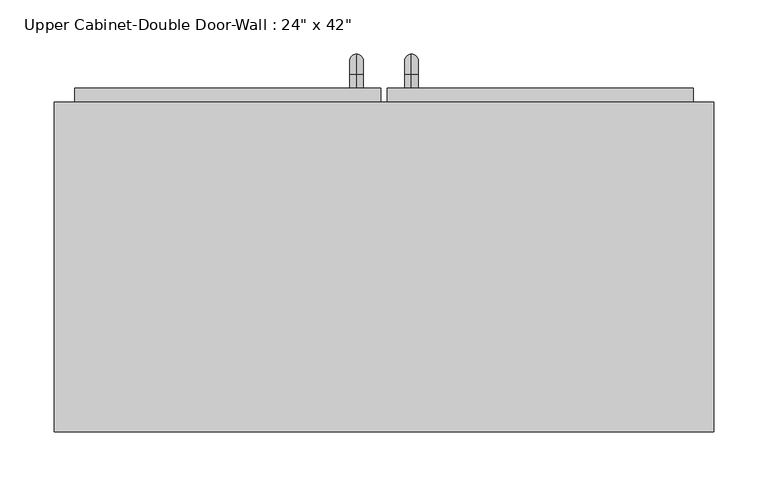
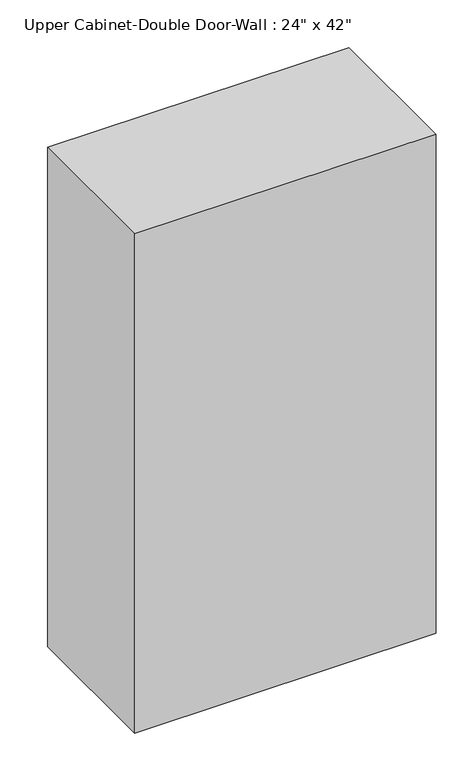
"""IFC4 building model written with IfcOpenShell, lengths in millimetres: furniture geometry."""

from ifc_helpers import new_model, si_unit, point, frame, origin, place, context, project, spatial, polyline, circle_curve, ellipse_curve, trimmed, outline, extrude, faceted_brep, source, transform, mapped, element, save
from ifc_brep_helpers import plane_surface, cylinder_surface, revolved_surface, advanced_brep


def furniture_378d84b8(model_context):
    return source(origin(), model_context, "Body", "SolidModel", [
        faceted_brep([(-275.0288372, 80.9625, 2438.4), (-275.0288372, 80.9625, 1371.6), (334.5711628, 80.9625, 1371.6), (334.5711628, 80.9625, 2438.4), (-275.0288372, 385.7625, 2438.4), (334.5711628, 385.7625, 2438.4), (334.5711628, 385.7625, 1371.6), (-275.0288372, 385.7625, 1371.6), (-255.9788372, 385.7625, 2419.35), (-255.9788372, 385.7625, 1390.65), (315.5211628, 385.7625, 1390.65), (315.5211628, 385.7625, 2419.35), (315.5211628, 100.0125, 2419.35), (-255.9788372, 100.0125, 2419.35), (315.5211628, 100.0125, 1390.65), (-255.9788372, 100.0125, 1390.65)], [[[0, 1, 2, 3]], [[4, 5, 6, 7], [8, 9, 10, 11]], [[1, 0, 4, 7]], [[2, 1, 7, 6]], [[3, 2, 6, 5]], [[0, 3, 5, 4]], [[8, 11, 12, 13]], [[11, 10, 14, 12]], [[10, 9, 15, 14]], [[9, 8, 13, 15]], [[13, 12, 14, 15]]]),
        advanced_brep(
        [(55.1711628, 398.4625, 1517.65), (55.1711628, 398.4625, 1530.35), (55.1711628, 411.1625, 1517.65), (55.1711628, 411.1625, 1530.35), (55.1711628, 430.2125, 1511.3), (55.1711628, 417.5125, 1511.3), (55.1711628, 417.5125, 1435.1), (55.1711628, 430.2125, 1435.1), (55.1711628, 411.1625, 1416.05), (55.1711628, 411.1625, 1428.75), (55.1711628, 398.4625, 1428.75), (55.1711628, 398.4625, 1416.05)],
        [
            (0, 1, circle_curve(frame((55.1711628, 398.4625, 1524.0), z_axis=(0.0, -1.0, 0.0), x_axis=(0.0, 0.0, -1.0)), 6.35)),
            (1, 0, circle_curve(frame((55.1711628, 398.4625, 1524.0), z_axis=(0.0, -1.0, 0.0), x_axis=(0.0, 0.0, -1.0)), 6.35)),
            (0, 2),
            (2, 3, circle_curve(frame((55.1711628, 411.1625, 1524.0), z_axis=(0.0, -1.0, 0.0), x_axis=(0.0, 0.0, -1.0)), 6.35)),
            (3, 1),
            (3, 2, circle_curve(frame((55.1711628, 411.1625, 1524.0), z_axis=(0.0, -1.0, 0.0), x_axis=(0.0, 0.0, -1.0)), 6.35)),
            (4, 3, circle_curve(frame((55.1711628, 411.1625, 1511.3), z_axis=(1.0, 0.0, 0.0), x_axis=(0.0, 0.0, 1.0)), 19.05)),
            (2, 5, circle_curve(frame((55.1711628, 411.1625, 1511.3), z_axis=(-1.0, 0.0, 0.0), x_axis=(0.0, 0.0, 1.0)), 6.35)),
            (5, 4, circle_curve(frame((55.1711628, 423.8625, 1511.3), z_axis=(0.0, 0.0, 1.0), x_axis=(0.0, -1.0, 0.0)), 6.35)),
            (4, 5, circle_curve(frame((55.1711628, 423.8625, 1511.3), z_axis=(0.0, 0.0, 1.0), x_axis=(0.0, -1.0, 0.0)), 6.35)),
            (5, 6),
            (6, 7, circle_curve(frame((55.1711628, 423.8625, 1435.1), z_axis=(0.0, 0.0, 1.0), x_axis=(0.0, -1.0, 0.0)), 6.35)),
            (7, 4),
            (7, 6, circle_curve(frame((55.1711628, 423.8625, 1435.1), z_axis=(0.0, 0.0, 1.0), x_axis=(0.0, -1.0, 0.0)), 6.35)),
            (8, 7, circle_curve(frame((55.1711628, 411.1625, 1435.1), z_axis=(1.0, 0.0, 0.0), x_axis=(0.0, 1.0, 0.0)), 19.05)),
            (6, 9, circle_curve(frame((55.1711628, 411.1625, 1435.1), z_axis=(-1.0, 0.0, 0.0), x_axis=(0.0, 1.0, 0.0)), 6.35)),
            (9, 8, circle_curve(frame((55.1711628, 411.1625, 1422.4), z_axis=(0.0, 1.0, 0.0), x_axis=(0.0, 0.0, 1.0)), 6.35)),
            (8, 9, circle_curve(frame((55.1711628, 411.1625, 1422.4), z_axis=(0.0, 1.0, 0.0), x_axis=(0.0, 0.0, 1.0)), 6.35)),
            (10, 11, circle_curve(frame((55.1711628, 398.4625, 1422.4), z_axis=(0.0, -1.0, 0.0), x_axis=(0.0, 0.0, 1.0)), 6.35)),
            (11, 10, circle_curve(frame((55.1711628, 398.4625, 1422.4), z_axis=(0.0, -1.0, 0.0), x_axis=(0.0, 0.0, 1.0)), 6.35)),
            (9, 10),
            (11, 8),
        ],
        [
            plane_surface(frame((48.8211628, 398.4625, 1524.0), z_axis=(0.0, -1.0, 0.0), x_axis=(0.0, 0.0, 1.0))),
            cylinder_surface(frame((55.1711628, 398.4625, 1524.0), z_axis=(0.0, -1.0, 0.0), x_axis=(0.0, 0.0, -1.0)), 6.35),
            revolved_surface(trimmed(ellipse_curve(frame((55.1711628, 411.1625, 1524.0), z_axis=(0.0, -1.0, 0.0), x_axis=(0.0, 0.0, -1.0)), 6.35, 6.35), [point((55.1711628, 411.1625, 1517.65))], [point((55.1711628, 411.1625, 1530.35))], True, "CARTESIAN"), (55.1711628, 411.1625, 1511.3), (-1.0, 0.0, 0.0)),
            revolved_surface(trimmed(ellipse_curve(frame((55.1711628, 411.1625, 1524.0), z_axis=(0.0, -1.0, 0.0), x_axis=(0.0, 0.0, -1.0)), 6.35, 6.35), [point((55.1711628, 411.1625, 1530.35))], [point((55.1711628, 411.1625, 1517.65))], True, "CARTESIAN"), (55.1711628, 411.1625, 1511.3), (-1.0, 0.0, 0.0)),
            cylinder_surface(frame((55.1711628, 423.8625, 1511.3), z_axis=(0.0, 0.0, 1.0), x_axis=(0.0, -1.0, 0.0)), 6.35),
            revolved_surface(trimmed(ellipse_curve(frame((55.1711628, 423.8625, 1435.1), z_axis=(0.0, 0.0, 1.0), x_axis=(0.0, -1.0, 0.0)), 6.35, 6.35), [point((55.1711628, 417.5125, 1435.1))], [point((55.1711628, 430.2125, 1435.1))], True, "CARTESIAN"), (55.1711628, 411.1625, 1435.1), (-1.0, 0.0, 0.0)),
            revolved_surface(trimmed(ellipse_curve(frame((55.1711628, 423.8625, 1435.1), z_axis=(0.0, 0.0, 1.0), x_axis=(0.0, -1.0, 0.0)), 6.35, 6.35), [point((55.1711628, 430.2125, 1435.1))], [point((55.1711628, 417.5125, 1435.1))], True, "CARTESIAN"), (55.1711628, 411.1625, 1435.1), (-1.0, 0.0, 0.0)),
            plane_surface(frame((48.8211628, 398.4625, 1422.4), z_axis=(0.0, -1.0, 0.0), x_axis=(0.0, 0.0, -1.0))),
            cylinder_surface(frame((55.1711628, 411.1625, 1422.4), z_axis=(0.0, 1.0, 0.0), x_axis=(0.0, 0.0, 1.0)), 6.35),
        ],
        [
            (0, [[1, 2]]),
            (1, [[-1, 3, 4, 5]]),
            (1, [[-2, -5, 6, -3]]),
            (2, [[7, -4, 8, 9]]),
            (3, [[-8, -6, -7, 10]]),
            (4, [[-9, 11, 12, 13]]),
            (4, [[-10, -13, 14, -11]]),
            (5, [[15, -12, 16, 17]]),
            (6, [[-16, -14, -15, 18]]),
            (7, [[19, 20]]),
            (8, [[-17, 21, -20, 22]]),
            (8, [[-18, -22, -19, -21]]),
        ],
    ),
        advanced_brep(
        [(4.3711628, 398.4625, 1517.65), (4.3711628, 398.4625, 1530.35), (4.3711628, 411.1625, 1517.65), (4.3711628, 411.1625, 1530.35), (4.3711628, 430.2125, 1511.3), (4.3711628, 417.5125, 1511.3), (4.3711628, 417.5125, 1435.1), (4.3711628, 430.2125, 1435.1), (4.3711628, 411.1625, 1416.05), (4.3711628, 411.1625, 1428.75), (4.3711628, 398.4625, 1428.75), (4.3711628, 398.4625, 1416.05)],
        [
            (0, 1, circle_curve(frame((4.3711628, 398.4625, 1524.0), z_axis=(0.0, -1.0, 0.0), x_axis=(0.0, 0.0, 1.0)), 6.35)),
            (1, 0, circle_curve(frame((4.3711628, 398.4625, 1524.0), z_axis=(0.0, -1.0, 0.0), x_axis=(0.0, 0.0, 1.0)), 6.35)),
            (0, 2),
            (2, 3, circle_curve(frame((4.3711628, 411.1625, 1524.0), z_axis=(0.0, -1.0, 0.0), x_axis=(0.0, 0.0, 1.0)), 6.35)),
            (3, 1),
            (3, 2, circle_curve(frame((4.3711628, 411.1625, 1524.0), z_axis=(0.0, -1.0, 0.0), x_axis=(0.0, 0.0, 1.0)), 6.35)),
            (4, 3, circle_curve(frame((4.3711628, 411.1625, 1511.3), z_axis=(1.0, 0.0, 0.0), x_axis=(0.0, 0.0, 1.0)), 19.05)),
            (2, 5, circle_curve(frame((4.3711628, 411.1625, 1511.3), z_axis=(-1.0, 0.0, 0.0), x_axis=(0.0, 0.0, 1.0)), 6.35)),
            (5, 4, circle_curve(frame((4.3711628, 423.8625, 1511.3), z_axis=(0.0, 0.0, 1.0), x_axis=(0.0, 1.0, 0.0)), 6.35)),
            (4, 5, circle_curve(frame((4.3711628, 423.8625, 1511.3), z_axis=(0.0, 0.0, 1.0), x_axis=(0.0, 1.0, 0.0)), 6.35)),
            (5, 6),
            (6, 7, circle_curve(frame((4.3711628, 423.8625, 1435.1), z_axis=(0.0, 0.0, 1.0), x_axis=(0.0, 1.0, 0.0)), 6.35)),
            (7, 4),
            (7, 6, circle_curve(frame((4.3711628, 423.8625, 1435.1), z_axis=(0.0, 0.0, 1.0), x_axis=(0.0, 1.0, 0.0)), 6.35)),
            (8, 7, circle_curve(frame((4.3711628, 411.1625, 1435.1), z_axis=(1.0, 0.0, 0.0), x_axis=(0.0, 1.0, 0.0)), 19.05)),
            (6, 9, circle_curve(frame((4.3711628, 411.1625, 1435.1), z_axis=(-1.0, 0.0, 0.0), x_axis=(0.0, 1.0, 0.0)), 6.35)),
            (9, 8, circle_curve(frame((4.3711628, 411.1625, 1422.4), z_axis=(0.0, 1.0, 0.0), x_axis=(0.0, 0.0, -1.0)), 6.35)),
            (8, 9, circle_curve(frame((4.3711628, 411.1625, 1422.4), z_axis=(0.0, 1.0, 0.0), x_axis=(0.0, 0.0, -1.0)), 6.35)),
            (10, 11, circle_curve(frame((4.3711628, 398.4625, 1422.4), z_axis=(0.0, -1.0, 0.0), x_axis=(0.0, 0.0, -1.0)), 6.35)),
            (11, 10, circle_curve(frame((4.3711628, 398.4625, 1422.4), z_axis=(0.0, -1.0, 0.0), x_axis=(0.0, 0.0, -1.0)), 6.35)),
            (9, 10),
            (11, 8),
        ],
        [
            plane_surface(frame((-1.9788372, 398.4625, 1524.0), z_axis=(0.0, -1.0, 0.0), x_axis=(0.0, 0.0, 1.0))),
            cylinder_surface(frame((4.3711628, 398.4625, 1524.0), z_axis=(0.0, -1.0, 0.0), x_axis=(0.0, 0.0, 1.0)), 6.35),
            revolved_surface(trimmed(ellipse_curve(frame((4.3711628, 411.1625, 1524.0), z_axis=(0.0, -1.0, 0.0), x_axis=(0.0, 0.0, 1.0)), 6.35, 6.35), [point((4.3711628, 411.1625, 1517.65))], [point((4.3711628, 411.1625, 1530.35))], True, "CARTESIAN"), (4.3711628, 411.1625, 1511.3), (-1.0, 0.0, 0.0)),
            revolved_surface(trimmed(ellipse_curve(frame((4.3711628, 411.1625, 1524.0), z_axis=(0.0, -1.0, 0.0), x_axis=(0.0, 0.0, 1.0)), 6.35, 6.35), [point((4.3711628, 411.1625, 1530.35))], [point((4.3711628, 411.1625, 1517.65))], True, "CARTESIAN"), (4.3711628, 411.1625, 1511.3), (-1.0, 0.0, 0.0)),
            cylinder_surface(frame((4.3711628, 423.8625, 1511.3), z_axis=(0.0, 0.0, 1.0), x_axis=(0.0, 1.0, 0.0)), 6.35),
            revolved_surface(trimmed(ellipse_curve(frame((4.3711628, 423.8625, 1435.1), z_axis=(0.0, 0.0, 1.0), x_axis=(0.0, 1.0, 0.0)), 6.35, 6.35), [point((4.3711628, 417.5125, 1435.1))], [point((4.3711628, 430.2125, 1435.1))], True, "CARTESIAN"), (4.3711628, 411.1625, 1435.1), (-1.0, 0.0, 0.0)),
            revolved_surface(trimmed(ellipse_curve(frame((4.3711628, 423.8625, 1435.1), z_axis=(0.0, 0.0, 1.0), x_axis=(0.0, 1.0, 0.0)), 6.35, 6.35), [point((4.3711628, 430.2125, 1435.1))], [point((4.3711628, 417.5125, 1435.1))], True, "CARTESIAN"), (4.3711628, 411.1625, 1435.1), (-1.0, 0.0, 0.0)),
            plane_surface(frame((-1.9788372, 398.4625, 1422.4), z_axis=(0.0, -1.0, 0.0), x_axis=(0.0, 0.0, -1.0))),
            cylinder_surface(frame((4.3711628, 411.1625, 1422.4), z_axis=(0.0, 1.0, 0.0), x_axis=(0.0, 0.0, -1.0)), 6.35),
        ],
        [
            (0, [[1, 2]]),
            (1, [[-1, 3, 4, 5]]),
            (1, [[-2, -5, 6, -3]]),
            (2, [[7, -4, 8, 9]]),
            (3, [[-8, -6, -7, 10]]),
            (4, [[-9, 11, 12, 13]]),
            (4, [[-10, -13, 14, -11]]),
            (5, [[15, -12, 16, 17]]),
            (6, [[-16, -14, -15, 18]]),
            (7, [[19, 20]]),
            (8, [[-17, 21, -20, 22]]),
            (8, [[-18, -22, -19, -21]]),
        ],
    ),
        extrude(outline(polyline([(32.9461628, 398.4625), (315.5211628, 398.4625), (315.5211628, 366.7125), (32.9461628, 366.7125), (32.9461628, 398.4625)])), frame((0.0, 0.0, 1390.65), z_axis=(0.0, 0.0, 1.0), x_axis=(1.0, 0.0, 0.0)), (0.0, 0.0, 1.0), 1028.7),
        extrude(outline(polyline([(-255.9788372, 398.4625), (26.5961628, 398.4625), (26.5961628, 366.7125), (-255.9788372, 366.7125), (-255.9788372, 398.4625)])), frame((0.0, 0.0, 1390.65), z_axis=(0.0, 0.0, 1.0), x_axis=(1.0, 0.0, 0.0)), (0.0, 0.0, 1.0), 1028.7),
    ])


if __name__ == "__main__":
    model = new_model("IFC4")
    model_context = context("Model", 3, world=origin())
    ifc_project = project(units=[si_unit("LENGTHUNIT", "METRE", prefix="MILLI")], contexts=[model_context])
    site = spatial("IfcSite", under=ifc_project)
    building = spatial("IfcBuilding", under=site)
    placement = place(None, origin())
    furniture_shape = furniture_378d84b8(model_context)
    element("IfcFurniture", 1, ObjectType="Upper Cabinet-Double Door-Wall : 24\" x 42\"", at=placement, inside=building, context=model_context, shape_type="MappedRepresentation", body=[
        mapped(furniture_shape, transform((0.0, 0.0, 0.0), x_axis=(1.0, 0.0, 0.0), y_axis=(0.0, 1.0, 0.0), z_axis=(0.0, 0.0, 1.0))),
    ])
    save(model, "model.ifc")

# Revit data of these elements
# Type "Upper Cabinet-Double Door-Wall : 24\" x 42\""
#   COBie.Type.CreatedBy = "doug.wood@us.ibm.com"
#   COBie.Type.CreatedOn = "2016-04-14T02:07:23"
#   COBie.Type.Name = "Casework_Upper Cabinet-Double Door-Wall_24\" x 42\""
#   COBie.Type.Category = "23-40 35 17 47 11 : Kitchen Casework"
#   COBie.Type.Description = "Upper Cabinet-Double Door-Wall_24\" x 42\""
#   COBie.Type.Manufacturer = ""
#   COBie.Type.ModelNumber = ""
#   Assembly Code = "C1030410"
#   COBie.Type.ReplacementCost = 0
#   Depth = 1' - 0"
#   Height = 3' - 6"
#   Top Of Cabinet = 8' - 0"
#   Width = 2' - 0"
#   COBie.Type = no
#   Cabinet Material = none
#   Door/Drawer Material = none
#   Handle Material = Cabinets - Handles
# Element 1 (IfcFurniture, "Upper Cabinet-Double Door-Wall : 24\" x 42\"")
#   Materials on its faces: "Cabinets - Handles", "Cabinets"
# Materials
#   "Cabinets - Handles": class "Metal", colour RGB 57 57 57, transparency 0
#   "Cabinets": class "Miscellaneous", colour RGB 249 249 249, transparency 0
